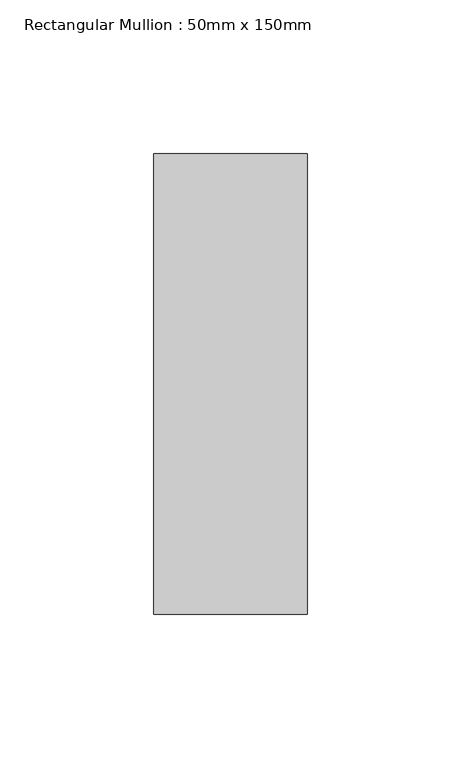
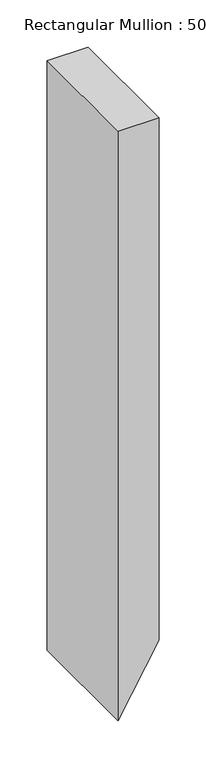
"""IFC4 building model written with IfcOpenShell, lengths in millimetres: member geometry, Rectangular Mullion : 50mm x 150mm."""

import ifcopenshell
import ifcopenshell.guid

model = None  # the IFC model being written
_history = None  # IfcOwnerHistory: only IFC2X3 demands one
_inside = {}  # id of a spatial element -> (the spatial element, [elements in it])
_under = {}  # id of a project, library or spatial element -> (it, [spatial elements below it])
_declared = {}  # id of a project -> (the project, [libraries it declares])
_typed = {}  # id of a type object -> (the type object, [elements of that type])
_made_of = {}  # id of a material, layer set ... -> (it, [elements and type objects made of it])


def new_model(schema):
    """Start an empty IFC model of exactly this schema.

    Asked for "IFC4X3", IfcOpenShell would pick the latest addendum, in which some entities
    have other attributes; the version numbers below select the first issue.
    IFC2X3 requires an IfcOwnerHistory on every rooted entity: one is made here for all.
    """
    global model, _history
    if schema == "IFC4X3":
        model = ifcopenshell.file(schema_version=(4, 3, 0, 0))
    else:
        model = ifcopenshell.file(schema=schema)
    _inside.clear()
    _under.clear()
    _declared.clear()
    _typed.clear()
    _made_of.clear()
    _history = None
    if model.schema == "IFC2X3":
        org = make("IfcOrganization", Name="unknown")
        user = make(
            "IfcPersonAndOrganization",
            ThePerson=make("IfcPerson", FamilyName="unknown"),
            TheOrganization=org,
        )
        app = make(
            "IfcApplication",
            ApplicationDeveloper=org,
            Version="unknown",
            ApplicationFullName="unknown",
            ApplicationIdentifier="unknown",
        )
        _history = make(
            "IfcOwnerHistory",
            OwningUser=user,
            OwningApplication=app,
            ChangeAction="ADDED",
            CreationDate=0,
        )
    return model


def make(cls, **values):
    """One entity of the class cls with the attributes given. An attribute that is None is left unset."""
    return model.create_entity(
        cls, **{name: value for name, value in values.items() if value is not None}
    )


def rooted(cls, **values):
    """An entity with a GlobalId (a new one), such as an element, a storey or a relation."""
    return make(cls, GlobalId=ifcopenshell.guid.new(), OwnerHistory=_history, **values)


def si_unit(unit_type, name, prefix=None):
    """IfcSIUnit, for example si_unit("LENGTHUNIT", "METRE", prefix="MILLI")."""
    return make("IfcSIUnit", UnitType=unit_type, Prefix=prefix, Name=name)


def assignment(units):
    """IfcUnitAssignment: the units of a project."""
    return None if units is None else make("IfcUnitAssignment", Units=units)


def point(xyz):
    """IfcCartesianPoint."""
    return None if xyz is None else make("IfcCartesianPoint", Coordinates=xyz)


def direction(xyz):
    """IfcDirection."""
    return None if xyz is None else make("IfcDirection", DirectionRatios=xyz)


def frame(location, z_axis=None, x_axis=None):
    """IfcAxis2Placement3D, a coordinate frame: its origin and axes. An axis left out is left unset."""
    return make(
        "IfcAxis2Placement3D",
        Location=point(location),
        Axis=direction(z_axis),
        RefDirection=direction(x_axis),
    )


def origin():
    """The frame at (0, 0, 0) with its axes left unset."""
    return frame((0.0, 0.0, 0.0))


def place(relative_to, where):
    """IfcLocalPlacement: puts the frame where relative to a parent placement (None: the world)."""
    return make(
        "IfcLocalPlacement", PlacementRelTo=relative_to, RelativePlacement=where
    )


def context(
    kind, dimensions, precision=None, world=None, true_north=None, identifier=None
):
    """IfcGeometricRepresentationContext, for example the 3D "Model" context."""
    return make(
        "IfcGeometricRepresentationContext",
        ContextIdentifier=identifier,
        ContextType=kind,
        CoordinateSpaceDimension=dimensions,
        Precision=precision,
        WorldCoordinateSystem=world,
        TrueNorth=true_north,
    )


def project(units=None, contexts=None):
    """IfcProject with its units and contexts."""
    return rooted(
        "IfcProject",
        Name="project",
        RepresentationContexts=contexts,
        UnitsInContext=assignment(units),
    )


def spatial(cls, under=None, at=None, **own):
    """A site, building, storey or space (cls), placed at a placement, below another one or the project."""
    s = rooted(cls, ObjectPlacement=at, **own)
    if under is not None:
        _under.setdefault(under.id(), (under, []))[1].append(s)
    return s


def polyline(points):
    """IfcPolyline through the points."""
    return make("IfcPolyline", Points=[point(p) for p in points])


def outline(outer, holes=None, kind="AREA"):
    """IfcArbitraryClosedProfileDef: a profile drawn as a closed curve; with holes, ...WithVoids."""
    if holes is None:
        return make("IfcArbitraryClosedProfileDef", ProfileType=kind, OuterCurve=outer)
    return make(
        "IfcArbitraryProfileDefWithVoids",
        ProfileType=kind,
        OuterCurve=outer,
        InnerCurves=holes,
    )


def extrude(swept, where, along, depth):
    """IfcExtrudedAreaSolid: the profile swept, set in the frame where, extruded along a direction by depth."""
    return make(
        "IfcExtrudedAreaSolid",
        SweptArea=swept,
        Position=where,
        ExtrudedDirection=direction(along),
        Depth=depth,
    )


def shape(context_of_items, identifier, shape_type, items):
    """IfcShapeRepresentation: the items that make up one representation, for example the "Body"."""
    return make(
        "IfcShapeRepresentation",
        ContextOfItems=context_of_items,
        RepresentationIdentifier=identifier,
        RepresentationType=shape_type,
        Items=items,
    )


def source(mapping_origin, context_of_items, identifier, shape_type, items):
    """IfcRepresentationMap: a shape defined once, which mapped items show again and again."""
    return make(
        "IfcRepresentationMap",
        MappingOrigin=mapping_origin,
        MappedRepresentation=shape(context_of_items, identifier, shape_type, items),
    )


def transform(
    local_origin,
    x_axis=None,
    y_axis=None,
    z_axis=None,
    scale=None,
    scale2=None,
    scale3=None,
    uniform=True,
):
    """IfcCartesianTransformationOperator3D, or its non-uniform kind. x_axis, y_axis, z_axis: its Axis1, 2, 3."""
    if uniform:
        return make(
            "IfcCartesianTransformationOperator3D",
            Axis1=direction(x_axis),
            Axis2=direction(y_axis),
            LocalOrigin=point(local_origin),
            Scale=scale,
            Axis3=direction(z_axis),
        )
    return make(
        "IfcCartesianTransformationOperator3DnonUniform",
        Axis1=direction(x_axis),
        Axis2=direction(y_axis),
        LocalOrigin=point(local_origin),
        Scale=scale,
        Axis3=direction(z_axis),
        Scale2=scale2,
        Scale3=scale3,
    )


def mapped(mapping_source, mapping_target):
    """IfcMappedItem: shows the shape of a source again, moved by a transform."""
    return make(
        "IfcMappedItem", MappingSource=mapping_source, MappingTarget=mapping_target
    )


def made_of(thing, what):
    """Note that an element or type object is made of a material, layer set ...; save() writes the relation."""
    if what is not None:
        _made_of.setdefault(what.id(), (what, []))[1].append(thing)
    return thing


def element(
    cls,
    number,
    at=None,
    inside=None,
    cuts=None,
    type_object=None,
    material=None,
    context=None,
    identifier="Body",
    shape_type=None,
    held_by="IfcProductDefinitionShape",
    body=None,
    shapes=None,
    **own,
):
    """One element of the class cls, such as IfcWall. Its Tag is "e" and its number.

    at: its placement. inside: the storey or other place that contains it. cuts: it is an
    opening in that element (IfcRelVoidsElement). A single representation is given by context,
    identifier, shape_type and body (its items); several are given by shapes. held_by: the class
    of the entity that holds the representations. save() writes the other relations.
    """
    e = rooted(cls, Tag="e%d" % number, ObjectPlacement=at, **own)
    if body is not None:
        shapes = [shape(context, identifier, shape_type, body)]
    if shapes is not None:
        e.Representation = make(held_by, Representations=shapes)
    if inside is not None:
        _inside.setdefault(inside.id(), (inside, []))[1].append(e)
    if cuts is not None:
        rooted(
            "IfcRelVoidsElement", RelatingBuildingElement=cuts, RelatedOpeningElement=e
        )
    if type_object is not None:
        _typed.setdefault(type_object.id(), (type_object, []))[1].append(e)
    return made_of(e, material)


def aggregate(whole, parts):
    """IfcRelAggregates: a whole, such as a stair, and the parts it consists of."""
    return rooted("IfcRelAggregates", RelatingObject=whole, RelatedObjects=parts)


def save(model, path):
    """Write the relations noted so far, then the file.

    IfcRelAggregates (storeys below a building ...), IfcRelContainedInSpatialStructure (elements
    in a storey), IfcRelDefinesByType, IfcRelAssociatesMaterial and IfcRelDeclares: one each for
    every whole, place, type object, material and project.
    """
    for whole, parts in _under.values():
        aggregate(whole, parts)
    for where, things in _inside.values():
        rooted(
            "IfcRelContainedInSpatialStructure",
            RelatedElements=things,
            RelatingStructure=where,
        )
    for kind, things in _typed.values():
        rooted("IfcRelDefinesByType", RelatedObjects=things, RelatingType=kind)
    for what, things in _made_of.values():
        rooted("IfcRelAssociatesMaterial", RelatedObjects=things, RelatingMaterial=what)
    for by, libraries in _declared.values():
        rooted("IfcRelDeclares", RelatingContext=by, RelatedDefinitions=libraries)
    model.write(path)


def rectangular_mullion_50mm_x_150mm_ac9de802(model_context):
    return source(origin(), model_context, "Body", "SweptSolid", [
        extrude(outline(polyline([(0.0, 25.0), (0.0, -25.0), (-761.4529717, -25.0), (-674.8504313, 25.0), (0.0, 25.0)])), frame((0.0, -75.0, 0.0), z_axis=(0.0, 1.0, 0.0), x_axis=(0.0, 0.0, 1.0)), (0.0, 0.0, 1.0), 150.0),
    ])


if __name__ == "__main__":
    model = new_model("IFC4")
    model_context = context("Model", 3, world=origin())
    ifc_project = project(units=[si_unit("LENGTHUNIT", "METRE", prefix="MILLI")], contexts=[model_context])
    site = spatial("IfcSite", under=ifc_project)
    building = spatial("IfcBuilding", under=site)
    placement = place(None, origin())
    rectangular_mullion_50mm_x_150mm_shape = rectangular_mullion_50mm_x_150mm_ac9de802(model_context)
    element("IfcMember", 1, ObjectType="Rectangular Mullion : 50mm x 150mm", at=placement, inside=building, context=model_context, shape_type="MappedRepresentation", body=[
        mapped(rectangular_mullion_50mm_x_150mm_shape, transform((0.0, 0.0, 0.0), x_axis=(1.0, 0.0, 0.0), y_axis=(0.0, 1.0, 0.0), z_axis=(0.0, 0.0, 1.0))),
    ])
    save(model, "model.ifc")

# Revit data of these elements
# Type "Rectangular Mullion : 50mm x 150mm"
#   built-in parameter 1007304 = 0.492126 (stored number, unit not read)
#   built-in parameter 1007301 = 0.082021 (stored number, unit not read)
#   built-in parameter 1007300 = 0.082021 (stored number, unit not read)
# Element 1 (IfcMember, "Rectangular Mullion : 50mm x 150mm")
#   Materials on its faces: "Aluminum"
# Materials
#   "Aluminum": class "Metal", colour RGB 247 247 247, transparency 0, Description = "Aluminum 6061", Cost = 0
